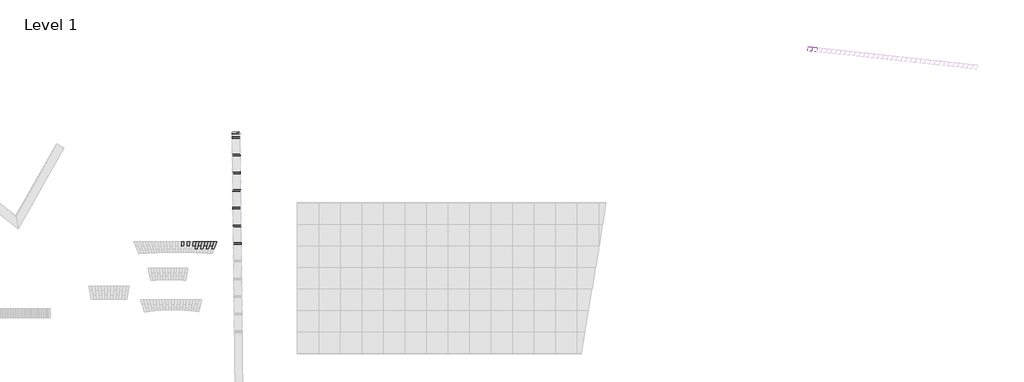
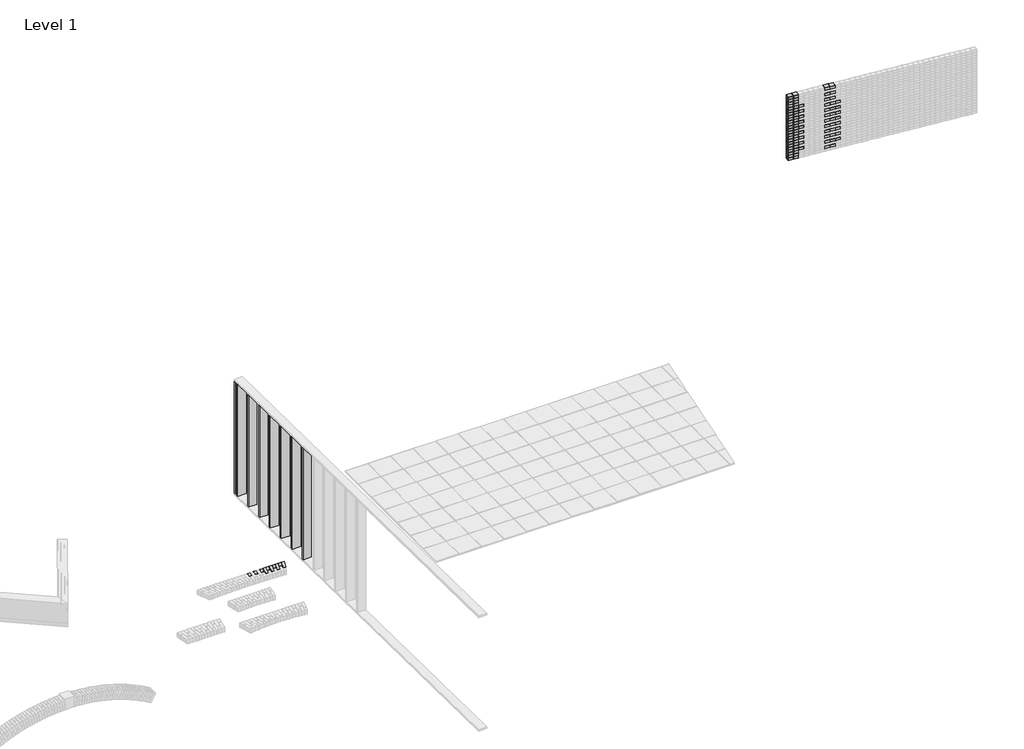
# One storey, part 11 of 18: 107 proxies.
# Revit data of these elements (continued)
# Type "00_GMA_hout : 184x38"
#   lengte [instance default] = 1198.641 mm
#   h = 38 mm
#   b = 184 mm
#   materiaal = 00_hout_vuren_generiek
#   PositionProfile [instance default] = 00_GMP_rectangle : TopLeft
#   Default Elevation = 0
# Type "00_GMA_hout : 38x184"
#   lengte [instance default] = 1198.641 mm
#   h = 184 mm
#   b = 38 mm
#   materiaal = 00_hout_vuren_generiek
#   PositionProfile [instance default] = 00_GMP_rectangle : TopLeft
#   Default Elevation = 0
# Type "00_GMA_steen_versie_6 : Geel"
#   Voegdikte = 95 mm
#   VoegTovSteen = -5 mm
#   StootvoegLinksHalfOnder [instance default] = 5 mm
#   StootvoegLinksHalfBoven [instance default] = 5 mm
#   StootVoegRechtsHalfOnder [instance default] = 5 mm
#   StootVoegRechtsHalfBoven [instance default] = 5 mm
#   StootVoegBreedteRechts [instance default] = 10 mm
#   StootVoegBreedteLinks [instance default] = 10 mm
#   Steendikte = 100 mm
#   LintVoegOnderHalf [instance default] = 0 mm
#   LintVoegOnder [instance default] = 0 mm
#   LintVoegBovenHalf [instance default] = 5 mm
#   LintVoegBoven [instance default] = 10 mm
#   materiaal = 21_steen_geel
#   MateriaalVoeg = 20_voeg
#   Default Elevation = 0
# Type "00_GMA_steen_versie_6 : Rood"
#   Voegdikte = 95 mm
#   VoegTovSteen = -5 mm
#   StootvoegLinksHalfOnder [instance default] = 5 mm
#   StootvoegLinksHalfBoven [instance default] = 5 mm
#   StootVoegRechtsHalfOnder [instance default] = 5 mm
#   StootVoegRechtsHalfBoven [instance default] = 5 mm
#   StootVoegBreedteRechts [instance default] = 10 mm
#   StootVoegBreedteLinks [instance default] = 10 mm
#   Steendikte = 100 mm
#   LintVoegOnderHalf [instance default] = 0 mm
#   LintVoegOnder [instance default] = 0 mm
#   LintVoegBovenHalf [instance default] = 5 mm
#   LintVoegBoven [instance default] = 10 mm
#   materiaal = 21_steen_rood
#   MateriaalVoeg = 20_voeg
#   Default Elevation = 0
# Type "00_GMA_steen_versie_4 : Steen Boven"
#   StootVoegHalfBoven [instance default] = 5 mm
#   StootVoegHalf [instance default] = 5 mm
#   StootVoegBreedteOnder = 10 mm
#   StootVoegBreedteBoven = 10 mm
#   Steendikte = 100 mm
#   LintVoegOnderHalf = 5 mm
#   LintVoegOnder = 10 mm
#   LintVoegBovenHalf = 0 mm
#   LintVoegBoven = 0 mm
#   materiaal = none
#   MateriaalVoeg = none
#   Default Elevation = 0
# Element 1 (IfcBuildingElementProxy, "00_GMA_hout : 184x38")
#   PositionProfile = 00_GMP_rectangle : TopRight
#   Phase Created = New Construction
#   Materials on its faces: "00_hout_vuren_generiek"
# Elements 2, 3, 4, 5, 6, 7, 8 (IfcBuildingElementProxy, "00_GMA_hout : 38x184")
#   PositionProfile = 00_GMP_rectangle : TopLeft
#   Phase Created = New Construction
#   Materials on its faces: "00_hout_vuren_generiek"
# Elements 9, 10, 11, 12, 13, 14, 15, 16, 17, 18, 19, 20, 21, 22, 23, 24, 25, 26, 27, 28, 29, 30, 31, 32, 33, 34, 35, 36, 37, 38, 39, 40, 41, 42, 43, 44, 45, 46, 47, 48, 49 (IfcBuildingElementProxy, "00_GMA_steen_versie_6 : Geel")
#   StootvoegLinksHalfOnder = 0 mm
#   StootvoegLinksHalfBoven = 0 mm
#   StootVoegRechtsHalfOnder = 5 mm
#   StootVoegRechtsHalfBoven = 5 mm
#   StootVoegBreedteRechts = 10 mm
#   StootVoegBreedteLinks = 0 mm
#   LintVoegOnderHalf = 5 mm
#   LintVoegOnder = 10 mm
#   LintVoegBovenHalf = 5 mm
#   LintVoegBoven = 10 mm
#   Phase Created = New Construction
#   Materials on its faces: "20_voeg", "21_steen_geel"
# Elements 50, 51, 52, 53, 54, 55, 56, 57, 58, 59, 60, 61, 62, 63, 64, 65, 66, 67, 68, 69, 70, 71, 72, 73 (IfcBuildingElementProxy, "00_GMA_steen_versie_6 : Geel")
#   StootvoegLinksHalfOnder = 5 mm
#   StootvoegLinksHalfBoven = 5 mm
#   StootVoegRechtsHalfOnder = 0 mm
#   StootVoegRechtsHalfBoven = 0 mm
#   StootVoegBreedteRechts = 0 mm
#   StootVoegBreedteLinks = 10 mm
#   LintVoegOnderHalf = 5 mm
#   LintVoegOnder = 10 mm
#   LintVoegBovenHalf = 5 mm
#   LintVoegBoven = 10 mm
#   Phase Created = New Construction
#   Materials on its faces: "20_voeg", "21_steen_geel"
# Elements 74, 75, 76, 77, 78, 79, 80, 81, 82, 83, 84, 85 (IfcBuildingElementProxy, "00_GMA_steen_versie_6 : Rood")
#   StootvoegLinksHalfOnder = 0 mm
#   StootvoegLinksHalfBoven = 0 mm
#   StootVoegRechtsHalfOnder = 5 mm
#   StootVoegRechtsHalfBoven = 5 mm
#   StootVoegBreedteRechts = 10 mm
#   StootVoegBreedteLinks = 0 mm
#   LintVoegOnderHalf = 5 mm
#   LintVoegOnder = 10 mm
#   LintVoegBovenHalf = 5 mm
#   LintVoegBoven = 10 mm
#   Phase Created = New Construction
#   Materials on its faces: "20_voeg", "21_steen_rood"
# Elements 86, 87, 88, 89, 90, 91, 92, 93, 94, 95, 96, 97 (IfcBuildingElementProxy, "00_GMA_steen_versie_6 : Rood")
#   StootvoegLinksHalfOnder = 5 mm
#   StootvoegLinksHalfBoven = 5 mm
#   StootVoegRechtsHalfOnder = 5 mm
#   StootVoegRechtsHalfBoven = 5 mm
#   StootVoegBreedteRechts = 10 mm
#   StootVoegBreedteLinks = 10 mm
#   LintVoegOnderHalf = 5 mm
#   LintVoegOnder = 10 mm
#   LintVoegBovenHalf = 5 mm
#   LintVoegBoven = 10 mm
#   Phase Created = New Construction
#   Materials on its faces: "20_voeg", "21_steen_rood"
# Elements 98, 99, 100, 101, 102, 103, 104, 105, 106, 107 (IfcBuildingElementProxy, "00_GMA_steen_versie_4 : Steen Boven")
#   StootVoegHalfBoven = 5 mm
#   StootVoegHalf = 5 mm
#   Phase Created = New Construction
# Materials
#   "00_hout_vuren_generiek": class "Wood", colour RGB 255 128 0, transparency 0, Manufacturer = "RevitGG", URL = "www.revitgg.nl", Description = "Hout, vuren, generiek", Cost = 0
#   "21_steen_geel": class "Unassigned", colour RGB 202 202 0, transparency 0, Cost = 0
#   "20_voeg": class "Concrete", colour RGB 86 86 86, transparency 0, Manufacturer = "RevitGG", URL = "www.revitgg.nl", Description = "zandcement, generiek materiaal", Cost = 0
#   "21_steen_rood": class "Unassigned", colour RGB 213 111 43, transparency 0, Cost = 0
